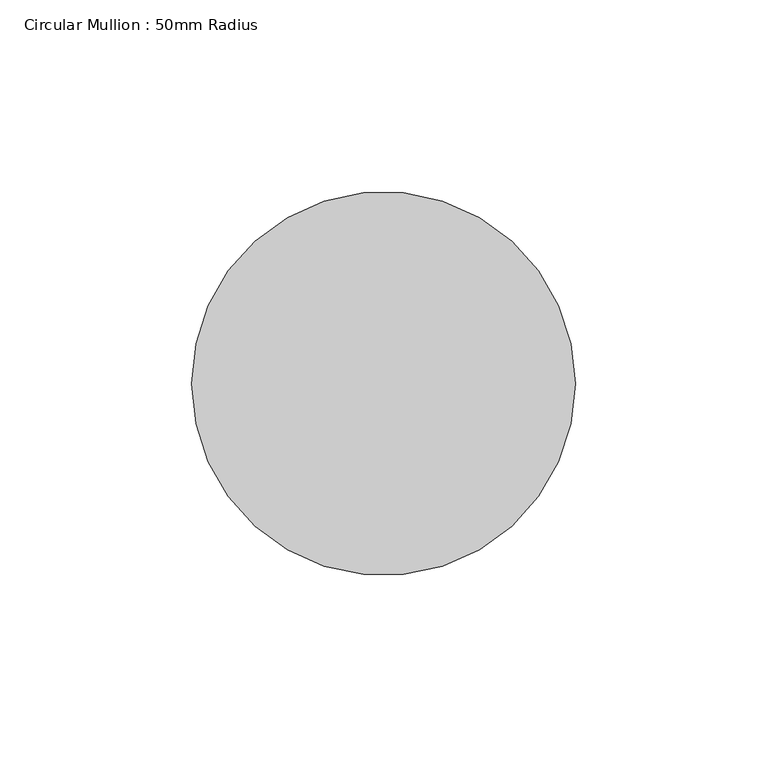
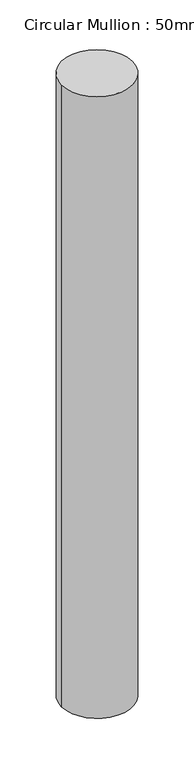
"""IFC4 building model written with IfcOpenShell, lengths in millimetres: member geometry, Circular Mullion : 50mm Radius."""

from ifc_helpers import new_model, si_unit, point, frame, origin, origin_2d, place, context, project, spatial, circle_curve, trimmed, segment, composite_curve, outline, extrude, source, transform, mapped, element, save


def circular_mullion_50mm_radius_ada7c6a0(model_context):
    return source(origin(), model_context, "Body", "SweptSolid", [
        extrude(outline(composite_curve([segment(trimmed(circle_curve(origin_2d(), 50.0), [point((50.0, 0.0))], [point((-50.0, 0.0))], False, "CARTESIAN"), True, "CONTINUOUS"), segment(trimmed(circle_curve(origin_2d(), 50.0), [point((-50.0, 0.0))], [point((50.0, 0.0))], False, "CARTESIAN"), True, "CONTINUOUS")], self_intersect=False)), frame((0.0, 0.0, -925.8564701), z_axis=(0.0, 0.0, 1.0), x_axis=(1.0, 0.0, 0.0)), (0.0, 0.0, 1.0), 925.8564701),
    ])


if __name__ == "__main__":
    model = new_model("IFC4")
    model_context = context("Model", 3, world=origin())
    ifc_project = project(units=[si_unit("LENGTHUNIT", "METRE", prefix="MILLI")], contexts=[model_context])
    site = spatial("IfcSite", under=ifc_project)
    building = spatial("IfcBuilding", under=site)
    placement = place(None, origin())
    circular_mullion_50mm_radius_shape = circular_mullion_50mm_radius_ada7c6a0(model_context)
    element("IfcMember", 1, ObjectType="Circular Mullion : 50mm Radius", at=placement, inside=building, context=model_context, shape_type="MappedRepresentation", body=[
        mapped(circular_mullion_50mm_radius_shape, transform((0.0, 0.0, 0.0), x_axis=(1.0, 0.0, 0.0), y_axis=(0.0, 1.0, 0.0), z_axis=(0.0, 0.0, 1.0))),
    ])
    save(model, "model.ifc")

# Revit data of these elements
# Type "Circular Mullion : 50mm Radius"
#   built-in parameter 1007350 = 0.164042 (stored number, unit not read)
# Element 1 (IfcMember, "Circular Mullion : 50mm Radius")
#   Materials on its faces: "Aluminium"
# Materials
#   "Aluminium": class "Metal", colour RGB 247 247 247, transparency 0, Description = "Aluminium 6061", Cost = 0
